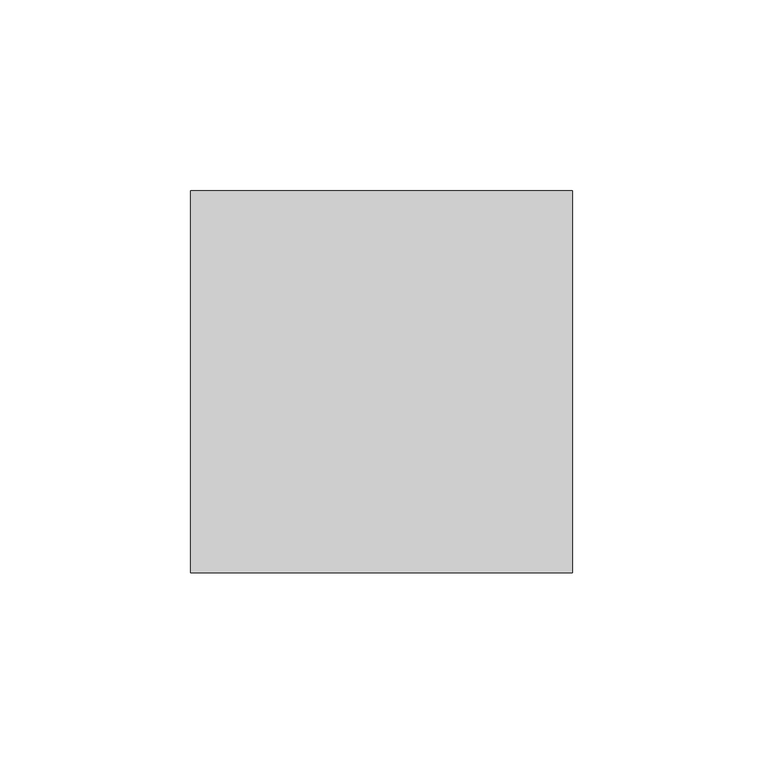
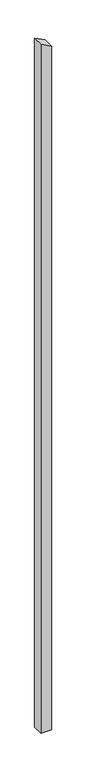
"""IFC4 building model written with IfcOpenShell, lengths in millimetres: column geometry, Holzstütze 159006 : Holzstütze 159006."""

import ifcopenshell
import ifcopenshell.guid

model = None  # the IFC model being written
_history = None  # IfcOwnerHistory: only IFC2X3 demands one
_inside = {}  # id of a spatial element -> (the spatial element, [elements in it])
_under = {}  # id of a project, library or spatial element -> (it, [spatial elements below it])
_declared = {}  # id of a project -> (the project, [libraries it declares])
_typed = {}  # id of a type object -> (the type object, [elements of that type])
_made_of = {}  # id of a material, layer set ... -> (it, [elements and type objects made of it])


def new_model(schema):
    """Start an empty IFC model of exactly this schema.

    Asked for "IFC4X3", IfcOpenShell would pick the latest addendum, in which some entities
    have other attributes; the version numbers below select the first issue.
    IFC2X3 requires an IfcOwnerHistory on every rooted entity: one is made here for all.
    """
    global model, _history
    if schema == "IFC4X3":
        model = ifcopenshell.file(schema_version=(4, 3, 0, 0))
    else:
        model = ifcopenshell.file(schema=schema)
    _inside.clear()
    _under.clear()
    _declared.clear()
    _typed.clear()
    _made_of.clear()
    _history = None
    if model.schema == "IFC2X3":
        org = make("IfcOrganization", Name="unknown")
        user = make(
            "IfcPersonAndOrganization",
            ThePerson=make("IfcPerson", FamilyName="unknown"),
            TheOrganization=org,
        )
        app = make(
            "IfcApplication",
            ApplicationDeveloper=org,
            Version="unknown",
            ApplicationFullName="unknown",
            ApplicationIdentifier="unknown",
        )
        _history = make(
            "IfcOwnerHistory",
            OwningUser=user,
            OwningApplication=app,
            ChangeAction="ADDED",
            CreationDate=0,
        )
    return model


def make(cls, **values):
    """One entity of the class cls with the attributes given. An attribute that is None is left unset."""
    return model.create_entity(
        cls, **{name: value for name, value in values.items() if value is not None}
    )


def rooted(cls, **values):
    """An entity with a GlobalId (a new one), such as an element, a storey or a relation."""
    return make(cls, GlobalId=ifcopenshell.guid.new(), OwnerHistory=_history, **values)


def si_unit(unit_type, name, prefix=None):
    """IfcSIUnit, for example si_unit("LENGTHUNIT", "METRE", prefix="MILLI")."""
    return make("IfcSIUnit", UnitType=unit_type, Prefix=prefix, Name=name)


def assignment(units):
    """IfcUnitAssignment: the units of a project."""
    return None if units is None else make("IfcUnitAssignment", Units=units)


def point(xyz):
    """IfcCartesianPoint."""
    return None if xyz is None else make("IfcCartesianPoint", Coordinates=xyz)


def direction(xyz):
    """IfcDirection."""
    return None if xyz is None else make("IfcDirection", DirectionRatios=xyz)


def frame(location, z_axis=None, x_axis=None):
    """IfcAxis2Placement3D, a coordinate frame: its origin and axes. An axis left out is left unset."""
    return make(
        "IfcAxis2Placement3D",
        Location=point(location),
        Axis=direction(z_axis),
        RefDirection=direction(x_axis),
    )


def origin():
    """The frame at (0, 0, 0) with its axes left unset."""
    return frame((0.0, 0.0, 0.0))


def place(relative_to, where):
    """IfcLocalPlacement: puts the frame where relative to a parent placement (None: the world)."""
    return make(
        "IfcLocalPlacement", PlacementRelTo=relative_to, RelativePlacement=where
    )


def context(
    kind, dimensions, precision=None, world=None, true_north=None, identifier=None
):
    """IfcGeometricRepresentationContext, for example the 3D "Model" context."""
    return make(
        "IfcGeometricRepresentationContext",
        ContextIdentifier=identifier,
        ContextType=kind,
        CoordinateSpaceDimension=dimensions,
        Precision=precision,
        WorldCoordinateSystem=world,
        TrueNorth=true_north,
    )


def project(units=None, contexts=None):
    """IfcProject with its units and contexts."""
    return rooted(
        "IfcProject",
        Name="project",
        RepresentationContexts=contexts,
        UnitsInContext=assignment(units),
    )


def spatial(cls, under=None, at=None, **own):
    """A site, building, storey or space (cls), placed at a placement, below another one or the project."""
    s = rooted(cls, ObjectPlacement=at, **own)
    if under is not None:
        _under.setdefault(under.id(), (under, []))[1].append(s)
    return s


def polyline(points):
    """IfcPolyline through the points."""
    return make("IfcPolyline", Points=[point(p) for p in points])


def outline(outer, holes=None, kind="AREA"):
    """IfcArbitraryClosedProfileDef: a profile drawn as a closed curve; with holes, ...WithVoids."""
    if holes is None:
        return make("IfcArbitraryClosedProfileDef", ProfileType=kind, OuterCurve=outer)
    return make(
        "IfcArbitraryProfileDefWithVoids",
        ProfileType=kind,
        OuterCurve=outer,
        InnerCurves=holes,
    )


def extrude(swept, where, along, depth):
    """IfcExtrudedAreaSolid: the profile swept, set in the frame where, extruded along a direction by depth."""
    return make(
        "IfcExtrudedAreaSolid",
        SweptArea=swept,
        Position=where,
        ExtrudedDirection=direction(along),
        Depth=depth,
    )


def shape(context_of_items, identifier, shape_type, items):
    """IfcShapeRepresentation: the items that make up one representation, for example the "Body"."""
    return make(
        "IfcShapeRepresentation",
        ContextOfItems=context_of_items,
        RepresentationIdentifier=identifier,
        RepresentationType=shape_type,
        Items=items,
    )


def source(mapping_origin, context_of_items, identifier, shape_type, items):
    """IfcRepresentationMap: a shape defined once, which mapped items show again and again."""
    return make(
        "IfcRepresentationMap",
        MappingOrigin=mapping_origin,
        MappedRepresentation=shape(context_of_items, identifier, shape_type, items),
    )


def transform(
    local_origin,
    x_axis=None,
    y_axis=None,
    z_axis=None,
    scale=None,
    scale2=None,
    scale3=None,
    uniform=True,
):
    """IfcCartesianTransformationOperator3D, or its non-uniform kind. x_axis, y_axis, z_axis: its Axis1, 2, 3."""
    if uniform:
        return make(
            "IfcCartesianTransformationOperator3D",
            Axis1=direction(x_axis),
            Axis2=direction(y_axis),
            LocalOrigin=point(local_origin),
            Scale=scale,
            Axis3=direction(z_axis),
        )
    return make(
        "IfcCartesianTransformationOperator3DnonUniform",
        Axis1=direction(x_axis),
        Axis2=direction(y_axis),
        LocalOrigin=point(local_origin),
        Scale=scale,
        Axis3=direction(z_axis),
        Scale2=scale2,
        Scale3=scale3,
    )


def mapped(mapping_source, mapping_target):
    """IfcMappedItem: shows the shape of a source again, moved by a transform."""
    return make(
        "IfcMappedItem", MappingSource=mapping_source, MappingTarget=mapping_target
    )


def made_of(thing, what):
    """Note that an element or type object is made of a material, layer set ...; save() writes the relation."""
    if what is not None:
        _made_of.setdefault(what.id(), (what, []))[1].append(thing)
    return thing


def element(
    cls,
    number,
    at=None,
    inside=None,
    cuts=None,
    type_object=None,
    material=None,
    context=None,
    identifier="Body",
    shape_type=None,
    held_by="IfcProductDefinitionShape",
    body=None,
    shapes=None,
    **own,
):
    """One element of the class cls, such as IfcWall. Its Tag is "e" and its number.

    at: its placement. inside: the storey or other place that contains it. cuts: it is an
    opening in that element (IfcRelVoidsElement). A single representation is given by context,
    identifier, shape_type and body (its items); several are given by shapes. held_by: the class
    of the entity that holds the representations. save() writes the other relations.
    """
    e = rooted(cls, Tag="e%d" % number, ObjectPlacement=at, **own)
    if body is not None:
        shapes = [shape(context, identifier, shape_type, body)]
    if shapes is not None:
        e.Representation = make(held_by, Representations=shapes)
    if inside is not None:
        _inside.setdefault(inside.id(), (inside, []))[1].append(e)
    if cuts is not None:
        rooted(
            "IfcRelVoidsElement", RelatingBuildingElement=cuts, RelatedOpeningElement=e
        )
    if type_object is not None:
        _typed.setdefault(type_object.id(), (type_object, []))[1].append(e)
    return made_of(e, material)


def aggregate(whole, parts):
    """IfcRelAggregates: a whole, such as a stair, and the parts it consists of."""
    return rooted("IfcRelAggregates", RelatingObject=whole, RelatedObjects=parts)


def save(model, path):
    """Write the relations noted so far, then the file.

    IfcRelAggregates (storeys below a building ...), IfcRelContainedInSpatialStructure (elements
    in a storey), IfcRelDefinesByType, IfcRelAssociatesMaterial and IfcRelDeclares: one each for
    every whole, place, type object, material and project.
    """
    for whole, parts in _under.values():
        aggregate(whole, parts)
    for where, things in _inside.values():
        rooted(
            "IfcRelContainedInSpatialStructure",
            RelatedElements=things,
            RelatingStructure=where,
        )
    for kind, things in _typed.values():
        rooted("IfcRelDefinesByType", RelatedObjects=things, RelatingType=kind)
    for what, things in _made_of.values():
        rooted("IfcRelAssociatesMaterial", RelatedObjects=things, RelatingMaterial=what)
    for by, libraries in _declared.values():
        rooted("IfcRelDeclares", RelatingContext=by, RelatedDefinitions=libraries)
    model.write(path)


def column_1fc37466(model_context):
    return source(origin(), model_context, "Body", "SweptSolid", [
        extrude(outline(polyline([(-500.0, 174197.7593015), (-500.0, 174297.7593015), (6345.7118258, 174297.7593015), (6396.6643707, 174197.7593015), (-500.0, 174197.7593015)])), frame((0.0, 47884.7962965, 0.0), z_axis=(0.0, 1.0, 0.0), x_axis=(0.0, 0.0, 1.0)), (0.0, 0.0, 1.0), 100.0),
    ])


if __name__ == "__main__":
    model = new_model("IFC4")
    model_context = context("Model", 3, world=origin())
    ifc_project = project(units=[si_unit("LENGTHUNIT", "METRE", prefix="MILLI")], contexts=[model_context])
    site = spatial("IfcSite", under=ifc_project)
    building = spatial("IfcBuilding", under=site)
    placement = place(None, origin())
    column_shape = column_1fc37466(model_context)
    element("IfcColumn", 1, ObjectType="Holzstütze 159006 : Holzstütze 159006", at=placement, inside=building, context=model_context, shape_type="MappedRepresentation", body=[
        mapped(column_shape, transform((0.0, 0.0, 0.0), x_axis=(1.0, 0.0, 0.0), y_axis=(0.0, 1.0, 0.0), z_axis=(0.0, 0.0, 1.0))),
    ])
    save(model, "model.ifc")

# Revit data of these elements
# Type "Holzstütze 159006 : Holzstütze 159006"
#   Abrechnungsart = "m"
#   Allright_Bauteil_ID = "0152St 0000143382"
#   Bezeichnung = "Holzstütze"
#   Codetext = "ST-HOLZ\\"
#   Gewerk = "Zimmer- und Holzbauarbeiten"
#   Material = "Holz"
#   Objektname = "Stütze"
#   NameOverride = "Holzstütze"
#   Reference = "Holzstütze"
#   Status = "NEW"
#   ThermalTransmittance = 0.0000 BTU/(h·ft²·°F)
#   Roll = 0.00°
#   Slope = 0.00°
#   2D Interaktion = yes
#   IsExternal = yes
#   LoadBearing = yes
# Element 1 (IfcColumn, "Holzstütze 159006 : Holzstütze 159006")
#   Materials on its faces: "holzschalung"
# Materials
#   "holzschalung": class "Unassigned", colour RGB 128 128 128, transparency 0
